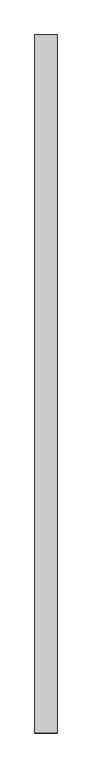
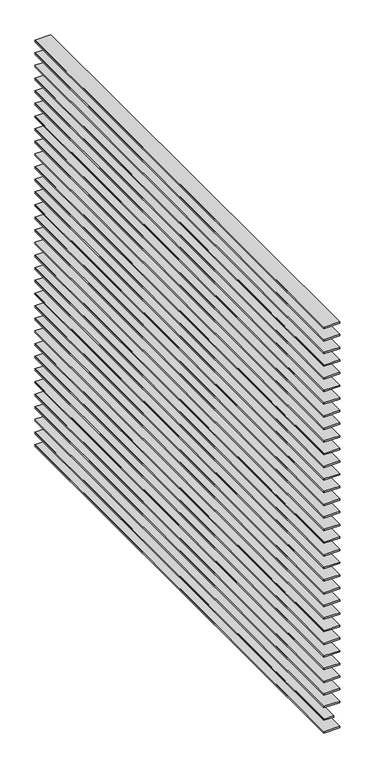
"""IFC4 building model written with IfcOpenShell, lengths in millimetres: proxy geometry, Brick 3:Brick 6179:305042 : Brick 3:Brick 6179:305042."""

from ifc_helpers import new_model, si_unit, point, frame, frame_2d, origin, place, context, project, spatial, polyline, circle_curve, trimmed, segment, composite_curve, outline, extrude, source, transform, mapped, element, save


def generic_models_00009414(model_context):
    return source(origin(), model_context, "Body", "SweptSolid", [
        extrude(outline(composite_curve([segment(polyline([(38976.8125, 14796.5703128), (38976.8125, 14860.0703128), (38982.7654111, 14860.0703128), (38982.7654111, 14796.5703128)]), True, "CONTINUOUS"), segment(trimmed(circle_curve(frame_2d((38979.7889555, 14793.8612881)), 4.0246867), [point((38982.7654111, 14796.5703128))], [point((38976.8125, 14796.5703128))], True, "CARTESIAN"), True, "CONTINUOUS")], self_intersect=False)), frame((0.0, 2495.6935399, 0.0), z_axis=(0.0, 1.0, 0.0), x_axis=(0.0, 0.0, 1.0)), (0.0, 0.0, 1.0), 2000.0),
        extrude(outline(composite_curve([segment(polyline([(38923.375, 14796.5703128), (38923.375, 14860.0703128), (38929.3279111, 14860.0703128), (38929.3279111, 14796.5703128)]), True, "CONTINUOUS"), segment(trimmed(circle_curve(frame_2d((38926.3514555, 14793.8612881)), 4.0246867), [point((38929.3279111, 14796.5703128))], [point((38923.375, 14796.5703128))], True, "CARTESIAN"), True, "CONTINUOUS")], self_intersect=False)), frame((0.0, 2495.6935399, 0.0), z_axis=(0.0, 1.0, 0.0), x_axis=(0.0, 0.0, 1.0)), (0.0, 0.0, 1.0), 2000.0),
        extrude(outline(composite_curve([segment(polyline([(38869.9375, 14796.5703128), (38869.9375, 14860.0703128), (38875.8904111, 14860.0703128), (38875.8904111, 14796.5703128)]), True, "CONTINUOUS"), segment(trimmed(circle_curve(frame_2d((38872.9139555, 14793.8612881)), 4.0246867), [point((38875.8904111, 14796.5703128))], [point((38869.9375, 14796.5703128))], True, "CARTESIAN"), True, "CONTINUOUS")], self_intersect=False)), frame((0.0, 2495.6935399, 0.0), z_axis=(0.0, 1.0, 0.0), x_axis=(0.0, 0.0, 1.0)), (0.0, 0.0, 1.0), 2000.0),
        extrude(outline(composite_curve([segment(polyline([(38816.5, 14796.5703128), (38816.5, 14860.0703128), (38822.4529111, 14860.0703128), (38822.4529111, 14796.5703128)]), True, "CONTINUOUS"), segment(trimmed(circle_curve(frame_2d((38819.4764555, 14793.8612881)), 4.0246867), [point((38822.4529111, 14796.5703128))], [point((38816.5, 14796.5703128))], True, "CARTESIAN"), True, "CONTINUOUS")], self_intersect=False)), frame((0.0, 2495.6935399, 0.0), z_axis=(0.0, 1.0, 0.0), x_axis=(0.0, 0.0, 1.0)), (0.0, 0.0, 1.0), 2000.0),
        extrude(outline(composite_curve([segment(polyline([(38763.0625, 14796.5703128), (38763.0625, 14860.0703128), (38769.0154111, 14860.0703128), (38769.0154111, 14796.5703128)]), True, "CONTINUOUS"), segment(trimmed(circle_curve(frame_2d((38766.0389555, 14793.8612881)), 4.0246867), [point((38769.0154111, 14796.5703128))], [point((38763.0625, 14796.5703128))], True, "CARTESIAN"), True, "CONTINUOUS")], self_intersect=False)), frame((0.0, 2495.6935399, 0.0), z_axis=(0.0, 1.0, 0.0), x_axis=(0.0, 0.0, 1.0)), (0.0, 0.0, 1.0), 2000.0),
        extrude(outline(composite_curve([segment(polyline([(38709.625, 14796.5703128), (38709.625, 14860.0703128), (38715.5779111, 14860.0703128), (38715.5779111, 14796.5703128)]), True, "CONTINUOUS"), segment(trimmed(circle_curve(frame_2d((38712.6014555, 14793.8612881)), 4.0246867), [point((38715.5779111, 14796.5703128))], [point((38709.625, 14796.5703128))], True, "CARTESIAN"), True, "CONTINUOUS")], self_intersect=False)), frame((0.0, 2495.6935399, 0.0), z_axis=(0.0, 1.0, 0.0), x_axis=(0.0, 0.0, 1.0)), (0.0, 0.0, 1.0), 2000.0),
        extrude(outline(composite_curve([segment(polyline([(38656.1875, 14796.5703128), (38656.1875, 14860.0703128), (38662.1404111, 14860.0703128), (38662.1404111, 14796.5703128)]), True, "CONTINUOUS"), segment(trimmed(circle_curve(frame_2d((38659.1639555, 14793.8612881)), 4.0246867), [point((38662.1404111, 14796.5703128))], [point((38656.1875, 14796.5703128))], True, "CARTESIAN"), True, "CONTINUOUS")], self_intersect=False)), frame((0.0, 2495.6935399, 0.0), z_axis=(0.0, 1.0, 0.0), x_axis=(0.0, 0.0, 1.0)), (0.0, 0.0, 1.0), 2000.0),
        extrude(outline(composite_curve([segment(polyline([(38602.75, 14796.5703128), (38602.75, 14860.0703128), (38608.7029111, 14860.0703128), (38608.7029111, 14796.5703128)]), True, "CONTINUOUS"), segment(trimmed(circle_curve(frame_2d((38605.7264555, 14793.8612881)), 4.0246867), [point((38608.7029111, 14796.5703128))], [point((38602.75, 14796.5703128))], True, "CARTESIAN"), True, "CONTINUOUS")], self_intersect=False)), frame((0.0, 2495.6935399, 0.0), z_axis=(0.0, 1.0, 0.0), x_axis=(0.0, 0.0, 1.0)), (0.0, 0.0, 1.0), 2000.0),
        extrude(outline(composite_curve([segment(polyline([(38549.3125, 14796.5703128), (38549.3125, 14860.0703128), (38555.2654111, 14860.0703128), (38555.2654111, 14796.5703128)]), True, "CONTINUOUS"), segment(trimmed(circle_curve(frame_2d((38552.2889555, 14793.8612881)), 4.0246867), [point((38555.2654111, 14796.5703128))], [point((38549.3125, 14796.5703128))], True, "CARTESIAN"), True, "CONTINUOUS")], self_intersect=False)), frame((0.0, 2495.6935399, 0.0), z_axis=(0.0, 1.0, 0.0), x_axis=(0.0, 0.0, 1.0)), (0.0, 0.0, 1.0), 2000.0),
        extrude(outline(composite_curve([segment(polyline([(38495.875, 14796.5703128), (38495.875, 14860.0703128), (38501.8279111, 14860.0703128), (38501.8279111, 14796.5703128)]), True, "CONTINUOUS"), segment(trimmed(circle_curve(frame_2d((38498.8514555, 14793.8612881)), 4.0246867), [point((38501.8279111, 14796.5703128))], [point((38495.875, 14796.5703128))], True, "CARTESIAN"), True, "CONTINUOUS")], self_intersect=False)), frame((0.0, 2495.6935399, 0.0), z_axis=(0.0, 1.0, 0.0), x_axis=(0.0, 0.0, 1.0)), (0.0, 0.0, 1.0), 2000.0),
        extrude(outline(composite_curve([segment(polyline([(38442.4375, 14796.5703128), (38442.4375, 14860.0703128), (38448.3904111, 14860.0703128), (38448.3904111, 14796.5703128)]), True, "CONTINUOUS"), segment(trimmed(circle_curve(frame_2d((38445.4139555, 14793.8612881)), 4.0246867), [point((38448.3904111, 14796.5703128))], [point((38442.4375, 14796.5703128))], True, "CARTESIAN"), True, "CONTINUOUS")], self_intersect=False)), frame((0.0, 2495.6935399, 0.0), z_axis=(0.0, 1.0, 0.0), x_axis=(0.0, 0.0, 1.0)), (0.0, 0.0, 1.0), 2000.0),
        extrude(outline(composite_curve([segment(polyline([(38389.0, 14796.5703128), (38389.0, 14860.0703128), (38394.9529111, 14860.0703128), (38394.9529111, 14796.5703128)]), True, "CONTINUOUS"), segment(trimmed(circle_curve(frame_2d((38391.9764555, 14793.8612881)), 4.0246867), [point((38394.9529111, 14796.5703128))], [point((38389.0, 14796.5703128))], True, "CARTESIAN"), True, "CONTINUOUS")], self_intersect=False)), frame((0.0, 2495.6935399, 0.0), z_axis=(0.0, 1.0, 0.0), x_axis=(0.0, 0.0, 1.0)), (0.0, 0.0, 1.0), 2000.0),
        extrude(outline(composite_curve([segment(polyline([(38335.5625, 14796.5703128), (38335.5625, 14860.0703128), (38341.5154111, 14860.0703128), (38341.5154111, 14796.5703128)]), True, "CONTINUOUS"), segment(trimmed(circle_curve(frame_2d((38338.5389555, 14793.8612881)), 4.0246867), [point((38341.5154111, 14796.5703128))], [point((38335.5625, 14796.5703128))], True, "CARTESIAN"), True, "CONTINUOUS")], self_intersect=False)), frame((0.0, 2495.6935399, 0.0), z_axis=(0.0, 1.0, 0.0), x_axis=(0.0, 0.0, 1.0)), (0.0, 0.0, 1.0), 2000.0),
        extrude(outline(composite_curve([segment(polyline([(38282.125, 14796.5703128), (38282.125, 14860.0703128), (38288.0779111, 14860.0703128), (38288.0779111, 14796.5703128)]), True, "CONTINUOUS"), segment(trimmed(circle_curve(frame_2d((38285.1014555, 14793.8612881)), 4.0246867), [point((38288.0779111, 14796.5703128))], [point((38282.125, 14796.5703128))], True, "CARTESIAN"), True, "CONTINUOUS")], self_intersect=False)), frame((0.0, 2495.6935399, 0.0), z_axis=(0.0, 1.0, 0.0), x_axis=(0.0, 0.0, 1.0)), (0.0, 0.0, 1.0), 2000.0),
        extrude(outline(composite_curve([segment(polyline([(38228.6875, 14796.5703128), (38228.6875, 14860.0703128), (38234.6404111, 14860.0703128), (38234.6404111, 14796.5703128)]), True, "CONTINUOUS"), segment(trimmed(circle_curve(frame_2d((38231.6639555, 14793.8612881)), 4.0246867), [point((38234.6404111, 14796.5703128))], [point((38228.6875, 14796.5703128))], True, "CARTESIAN"), True, "CONTINUOUS")], self_intersect=False)), frame((0.0, 2495.6935399, 0.0), z_axis=(0.0, 1.0, 0.0), x_axis=(0.0, 0.0, 1.0)), (0.0, 0.0, 1.0), 2000.0),
        extrude(outline(composite_curve([segment(polyline([(38175.25, 14796.5703128), (38175.25, 14860.0703128), (38181.2029111, 14860.0703128), (38181.2029111, 14796.5703128)]), True, "CONTINUOUS"), segment(trimmed(circle_curve(frame_2d((38178.2264555, 14793.8612881)), 4.0246867), [point((38181.2029111, 14796.5703128))], [point((38175.25, 14796.5703128))], True, "CARTESIAN"), True, "CONTINUOUS")], self_intersect=False)), frame((0.0, 2495.6935399, 0.0), z_axis=(0.0, 1.0, 0.0), x_axis=(0.0, 0.0, 1.0)), (0.0, 0.0, 1.0), 2000.0),
        extrude(outline(composite_curve([segment(polyline([(38121.8125, 14796.5703128), (38121.8125, 14860.0703128), (38127.7654111, 14860.0703128), (38127.7654111, 14796.5703128)]), True, "CONTINUOUS"), segment(trimmed(circle_curve(frame_2d((38124.7889555, 14793.8612881)), 4.0246867), [point((38127.7654111, 14796.5703128))], [point((38121.8125, 14796.5703128))], True, "CARTESIAN"), True, "CONTINUOUS")], self_intersect=False)), frame((0.0, 2495.6935399, 0.0), z_axis=(0.0, 1.0, 0.0), x_axis=(0.0, 0.0, 1.0)), (0.0, 0.0, 1.0), 2000.0),
        extrude(outline(composite_curve([segment(polyline([(38068.375, 14796.5703128), (38068.375, 14860.0703128), (38074.3279111, 14860.0703128), (38074.3279111, 14796.5703128)]), True, "CONTINUOUS"), segment(trimmed(circle_curve(frame_2d((38071.3514555, 14793.8612881)), 4.0246867), [point((38074.3279111, 14796.5703128))], [point((38068.375, 14796.5703128))], True, "CARTESIAN"), True, "CONTINUOUS")], self_intersect=False)), frame((0.0, 2495.6935399, 0.0), z_axis=(0.0, 1.0, 0.0), x_axis=(0.0, 0.0, 1.0)), (0.0, 0.0, 1.0), 2000.0),
        extrude(outline(composite_curve([segment(polyline([(38014.9375, 14796.5703128), (38014.9375, 14860.0703128), (38020.8904111, 14860.0703128), (38020.8904111, 14796.5703128)]), True, "CONTINUOUS"), segment(trimmed(circle_curve(frame_2d((38017.9139555, 14793.8612881)), 4.0246867), [point((38020.8904111, 14796.5703128))], [point((38014.9375, 14796.5703128))], True, "CARTESIAN"), True, "CONTINUOUS")], self_intersect=False)), frame((0.0, 2495.6935399, 0.0), z_axis=(0.0, 1.0, 0.0), x_axis=(0.0, 0.0, 1.0)), (0.0, 0.0, 1.0), 2000.0),
        extrude(outline(composite_curve([segment(polyline([(37961.5, 14796.5703128), (37961.5, 14860.0703128), (37967.4529111, 14860.0703128), (37967.4529111, 14796.5703128)]), True, "CONTINUOUS"), segment(trimmed(circle_curve(frame_2d((37964.4764555, 14793.8612881)), 4.0246867), [point((37967.4529111, 14796.5703128))], [point((37961.5, 14796.5703128))], True, "CARTESIAN"), True, "CONTINUOUS")], self_intersect=False)), frame((0.0, 2495.6935399, 0.0), z_axis=(0.0, 1.0, 0.0), x_axis=(0.0, 0.0, 1.0)), (0.0, 0.0, 1.0), 2000.0),
        extrude(outline(composite_curve([segment(polyline([(37908.0625, 14796.5703128), (37908.0625, 14860.0703128), (37914.0154111, 14860.0703128), (37914.0154111, 14796.5703128)]), True, "CONTINUOUS"), segment(trimmed(circle_curve(frame_2d((37911.0389555, 14793.8612881)), 4.0246867), [point((37914.0154111, 14796.5703128))], [point((37908.0625, 14796.5703128))], True, "CARTESIAN"), True, "CONTINUOUS")], self_intersect=False)), frame((0.0, 2495.6935399, 0.0), z_axis=(0.0, 1.0, 0.0), x_axis=(0.0, 0.0, 1.0)), (0.0, 0.0, 1.0), 2000.0),
        extrude(outline(composite_curve([segment(polyline([(37854.625, 14796.5703128), (37854.625, 14860.0703128), (37860.5779111, 14860.0703128), (37860.5779111, 14796.5703128)]), True, "CONTINUOUS"), segment(trimmed(circle_curve(frame_2d((37857.6014555, 14793.8612881)), 4.0246867), [point((37860.5779111, 14796.5703128))], [point((37854.625, 14796.5703128))], True, "CARTESIAN"), True, "CONTINUOUS")], self_intersect=False)), frame((0.0, 2495.6935399, 0.0), z_axis=(0.0, 1.0, 0.0), x_axis=(0.0, 0.0, 1.0)), (0.0, 0.0, 1.0), 2000.0),
        extrude(outline(composite_curve([segment(polyline([(37801.1875, 14796.5703128), (37801.1875, 14860.0703128), (37807.1404111, 14860.0703128), (37807.1404111, 14796.5703128)]), True, "CONTINUOUS"), segment(trimmed(circle_curve(frame_2d((37804.1639555, 14793.8612881)), 4.0246867), [point((37807.1404111, 14796.5703128))], [point((37801.1875, 14796.5703128))], True, "CARTESIAN"), True, "CONTINUOUS")], self_intersect=False)), frame((0.0, 2495.6935399, 0.0), z_axis=(0.0, 1.0, 0.0), x_axis=(0.0, 0.0, 1.0)), (0.0, 0.0, 1.0), 2000.0),
        extrude(outline(composite_curve([segment(polyline([(37747.75, 14796.5703128), (37747.75, 14860.0703128), (37753.7029111, 14860.0703128), (37753.7029111, 14796.5703128)]), True, "CONTINUOUS"), segment(trimmed(circle_curve(frame_2d((37750.7264555, 14793.8612881)), 4.0246867), [point((37753.7029111, 14796.5703128))], [point((37747.75, 14796.5703128))], True, "CARTESIAN"), True, "CONTINUOUS")], self_intersect=False)), frame((0.0, 2495.6935399, 0.0), z_axis=(0.0, 1.0, 0.0), x_axis=(0.0, 0.0, 1.0)), (0.0, 0.0, 1.0), 2000.0),
        extrude(outline(composite_curve([segment(polyline([(37694.3125, 14796.5703128), (37694.3125, 14860.0703128), (37700.2654111, 14860.0703128), (37700.2654111, 14796.5703128)]), True, "CONTINUOUS"), segment(trimmed(circle_curve(frame_2d((37697.2889555, 14793.8612881)), 4.0246867), [point((37700.2654111, 14796.5703128))], [point((37694.3125, 14796.5703128))], True, "CARTESIAN"), True, "CONTINUOUS")], self_intersect=False)), frame((0.0, 2495.6935399, 0.0), z_axis=(0.0, 1.0, 0.0), x_axis=(0.0, 0.0, 1.0)), (0.0, 0.0, 1.0), 2000.0),
        extrude(outline(composite_curve([segment(polyline([(37640.875, 14796.5703128), (37640.875, 14860.0703128), (37646.8279111, 14860.0703128), (37646.8279111, 14796.5703128)]), True, "CONTINUOUS"), segment(trimmed(circle_curve(frame_2d((37643.8514555, 14793.8612881)), 4.0246867), [point((37646.8279111, 14796.5703128))], [point((37640.875, 14796.5703128))], True, "CARTESIAN"), True, "CONTINUOUS")], self_intersect=False)), frame((0.0, 2495.6935399, 0.0), z_axis=(0.0, 1.0, 0.0), x_axis=(0.0, 0.0, 1.0)), (0.0, 0.0, 1.0), 2000.0),
        extrude(outline(composite_curve([segment(polyline([(37587.4375, 14796.5703128), (37587.4375, 14860.0703128), (37593.3904111, 14860.0703128), (37593.3904111, 14796.5703128)]), True, "CONTINUOUS"), segment(trimmed(circle_curve(frame_2d((37590.4139555, 14793.8612881)), 4.0246867), [point((37593.3904111, 14796.5703128))], [point((37587.4375, 14796.5703128))], True, "CARTESIAN"), True, "CONTINUOUS")], self_intersect=False)), frame((0.0, 2495.6935399, 0.0), z_axis=(0.0, 1.0, 0.0), x_axis=(0.0, 0.0, 1.0)), (0.0, 0.0, 1.0), 2000.0),
        extrude(outline(composite_curve([segment(polyline([(37534.0, 14796.5703128), (37534.0, 14860.0703128), (37539.9529111, 14860.0703128), (37539.9529111, 14796.5703128)]), True, "CONTINUOUS"), segment(trimmed(circle_curve(frame_2d((37536.9764555, 14793.8612881)), 4.0246867), [point((37539.9529111, 14796.5703128))], [point((37534.0, 14796.5703128))], True, "CARTESIAN"), True, "CONTINUOUS")], self_intersect=False)), frame((0.0, 2495.6935399, 0.0), z_axis=(0.0, 1.0, 0.0), x_axis=(0.0, 0.0, 1.0)), (0.0, 0.0, 1.0), 2000.0),
        extrude(outline(composite_curve([segment(polyline([(37480.5625, 14796.5703128), (37480.5625, 14860.0703128), (37486.5154111, 14860.0703128), (37486.5154111, 14796.5703128)]), True, "CONTINUOUS"), segment(trimmed(circle_curve(frame_2d((37483.5389555, 14793.8612881)), 4.0246867), [point((37486.5154111, 14796.5703128))], [point((37480.5625, 14796.5703128))], True, "CARTESIAN"), True, "CONTINUOUS")], self_intersect=False)), frame((0.0, 2495.6935399, 0.0), z_axis=(0.0, 1.0, 0.0), x_axis=(0.0, 0.0, 1.0)), (0.0, 0.0, 1.0), 2000.0),
        extrude(outline(composite_curve([segment(polyline([(37427.125, 14796.5703128), (37427.125, 14860.0703128), (37433.0779111, 14860.0703128), (37433.0779111, 14796.5703128)]), True, "CONTINUOUS"), segment(trimmed(circle_curve(frame_2d((37430.1014555, 14793.8612881)), 4.0246867), [point((37433.0779111, 14796.5703128))], [point((37427.125, 14796.5703128))], True, "CARTESIAN"), True, "CONTINUOUS")], self_intersect=False)), frame((0.0, 2495.6935399, 0.0), z_axis=(0.0, 1.0, 0.0), x_axis=(0.0, 0.0, 1.0)), (0.0, 0.0, 1.0), 2000.0),
        extrude(outline(composite_curve([segment(polyline([(37373.6875, 14796.5703128), (37373.6875, 14836.9038346), (37379.6404111, 14836.9038346), (37379.6404111, 14796.5703128)]), True, "CONTINUOUS"), segment(trimmed(circle_curve(frame_2d((37376.6639555, 14793.8612881)), 4.0246867), [point((37379.6404111, 14796.5703128))], [point((37373.6875, 14796.5703128))], True, "CARTESIAN"), True, "CONTINUOUS")], self_intersect=False)), frame((0.0, 2495.6935399, 0.0), z_axis=(0.0, 1.0, 0.0), x_axis=(0.0, 0.0, 1.0)), (0.0, 0.0, 1.0), 2000.0),
        extrude(outline(composite_curve([segment(polyline([(39030.25, 14796.5703128), (39030.25, 14860.0703128), (39036.2029111, 14860.0703128), (39036.2029111, 14796.5703128)]), True, "CONTINUOUS"), segment(trimmed(circle_curve(frame_2d((39033.2264555, 14793.8612881)), 4.0246867), [point((39036.2029111, 14796.5703128))], [point((39030.25, 14796.5703128))], True, "CARTESIAN"), True, "CONTINUOUS")], self_intersect=False)), frame((0.0, 2495.6935399, 0.0), z_axis=(0.0, 1.0, 0.0), x_axis=(0.0, 0.0, 1.0)), (0.0, 0.0, 1.0), 2000.0),
        extrude(outline(composite_curve([segment(polyline([(37320.25, 14796.5703128), (37320.25, 14860.0703128), (37326.2029111, 14860.0703128), (37326.2029111, 14796.5703128)]), True, "CONTINUOUS"), segment(trimmed(circle_curve(frame_2d((37323.2264555, 14793.8612881)), 4.0246867), [point((37326.2029111, 14796.5703128))], [point((37320.25, 14796.5703128))], True, "CARTESIAN"), True, "CONTINUOUS")], self_intersect=False)), frame((0.0, 2495.6935399, 0.0), z_axis=(0.0, 1.0, 0.0), x_axis=(0.0, 0.0, 1.0)), (0.0, 0.0, 1.0), 2000.0),
    ])


if __name__ == "__main__":
    model = new_model("IFC4")
    model_context = context("Model", 3, world=origin())
    ifc_project = project(units=[si_unit("LENGTHUNIT", "METRE", prefix="MILLI")], contexts=[model_context])
    site = spatial("IfcSite", under=ifc_project)
    building = spatial("IfcBuilding", under=site)
    placement = place(None, origin())
    generic_models_shape = generic_models_00009414(model_context)
    element("IfcBuildingElementProxy", 1, Name="Brick 3:Brick 6179:305042 : Brick 3:Brick 6179:305042", ObjectType="Brick 3:Brick 6179:305042 : Brick 3:Brick 6179:305042", at=placement, inside=building, context=model_context, shape_type="MappedRepresentation", body=[
        mapped(generic_models_shape, transform((0.0, 0.0, 0.0), x_axis=(1.0, 0.0, 0.0), y_axis=(0.0, 1.0, 0.0), z_axis=(0.0, 0.0, 1.0))),
    ])
    save(model, "model.ifc")

# Revit data of these elements
# Project information
#   IfcApplicationVersion = "2020"
#   IfcApplicationName = "Autodesk Revit 2020 (ENU)"
#   IfcSite GUID = "2PWCYz3SjEt8pmJZyx4El5"
#   IfcBuilding GUID = "2PWCYz3SjEt8pmJZyx4El6"
#   IfcProject GUID = "2PWCYz3SjEt8pmJZyx4El7"
#   IsLandmarked = "No"
#   NumberOfStoreys = "2"
#   Category = "Project Information"
#   NameOverride = "Default"
#   Project Issue Date = "Issue Date"
#   Project Status = "Project Status"
#   Client Name = "Owner"
#   Project Address = "Enter address here"
#   Project Name = "Project Name"
#   Project Number = "Project Number"
# Type "Brick 3:Brick 6179:305042 : Brick 3:Brick 6179:305042"
#   NameOverride = "Brick 3:Brick 6179:305042"
#   ObjectTypeOverride = "Brick 3:Brick 6179"
#   Reference = "Brick 6179"
#   Category = "Generic Models"
#   Tag = "305042"
# Element 1 (IfcBuildingElementProxy, "Brick 3:Brick 6179:305042 : Brick 3:Brick 6179:305042")
#   Materials on its faces: "MORTAR BED"
# Materials
#   "MORTAR BED": class "Unassigned", colour RGB 186 186 186, transparency 0, Cost = 0
